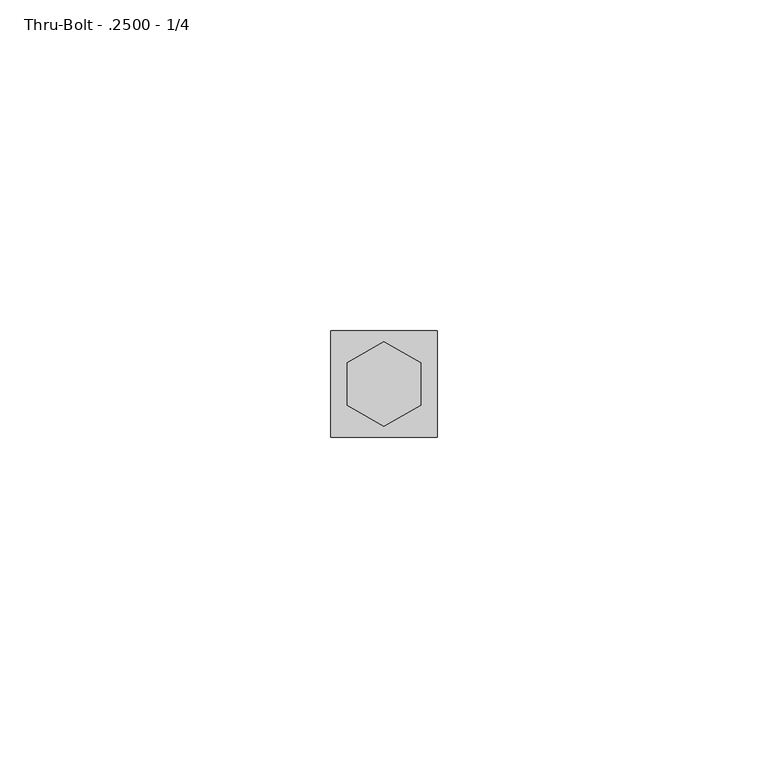
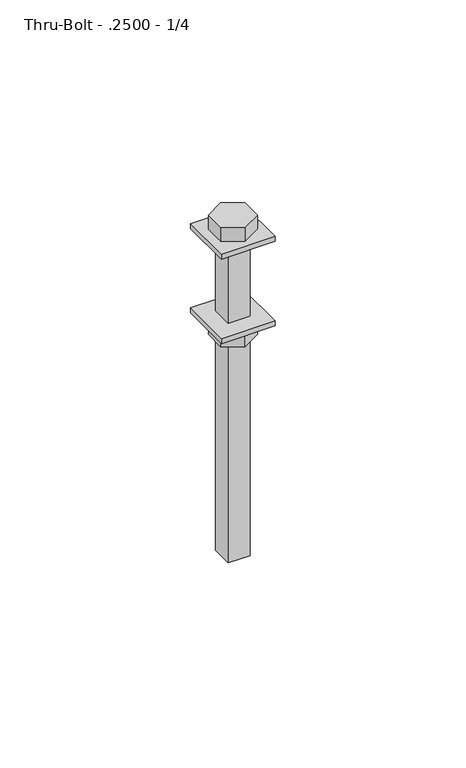
"""IFC4 building model written with IfcOpenShell, lengths in millimetres: fastener geometry, 060523 - W_P_C - Fastenings - Generic - SQUARE : Thru-Bolt - .2500 - 1/4."""

from ifc_helpers import new_model, si_unit, frame, origin, origin_with_axes, place, context, project, spatial, polyline, outline, extrude, source, transform, mapped, element, save


def thru_bolt_2500_1_4_f6ebfea6(model_context):
    return source(origin(), model_context, "Body", "SweptSolid", [
        extrude(outline(polyline([(-8.0645, -8.0645), (-8.0645, 8.0645), (8.0645, 8.0645), (8.0645, -8.0645), (-8.0645, -8.0645)])), origin_with_axes(), (0.0, 0.0, 1.0), 1.5875),
        extrude(outline(polyline([(-8.0645, -8.0645), (-8.0645, 8.0645), (8.0645, 8.0645), (8.0645, -8.0645), (-8.0645, -8.0645)])), frame((0.0, 0.0, -26.9875), z_axis=(0.0, 0.0, 1.0), x_axis=(1.0, 0.0, 0.0)), (0.0, 0.0, 1.0), 1.5875),
        extrude(outline(polyline([(-5.55625, -3.2079024), (-5.55625, 3.2079024), (0.0, 6.4158049), (5.55625, 3.2079024), (5.55625, -3.2079024), (0.0, -6.4158049), (-5.55625, -3.2079024)])), frame((0.0, 0.0, -31.75), z_axis=(0.0, 0.0, 1.0), x_axis=(1.0, 0.0, 0.0)), (0.0, 0.0, 1.0), 4.7625),
        extrude(outline(polyline([(-5.55625, 3.2079024), (0.0, 6.4158049), (5.55625, 3.2079024), (5.55625, -3.2079024), (0.0, -6.4158049), (-5.55625, -3.2079024), (-5.55625, 3.2079024)])), frame((0.0, 0.0, 1.5875), z_axis=(0.0, 0.0, 1.0), x_axis=(1.0, 0.0, 0.0)), (0.0, 0.0, 1.0), 4.7625),
        extrude(outline(polyline([(-3.302, 3.302), (3.302, 3.302), (3.302, -3.302), (-3.302, -3.302), (-3.302, 3.302)])), frame((0.0, 0.0, -101.6), z_axis=(0.0, 0.0, 1.0), x_axis=(1.0, 0.0, 0.0)), (0.0, 0.0, 1.0), 103.1875),
    ])


if __name__ == "__main__":
    model = new_model("IFC4")
    model_context = context("Model", 3, world=origin())
    ifc_project = project(units=[si_unit("LENGTHUNIT", "METRE", prefix="MILLI")], contexts=[model_context])
    site = spatial("IfcSite", under=ifc_project)
    building = spatial("IfcBuilding", under=site)
    placement = place(None, origin())
    thru_bolt_2500_1_4_shape = thru_bolt_2500_1_4_f6ebfea6(model_context)
    element("IfcFastener", 1, ObjectType="060523 - W_P_C - Fastenings - Generic - SQUARE : Thru-Bolt - .2500 - 1/4", at=placement, inside=building, context=model_context, shape_type="MappedRepresentation", body=[
        mapped(thru_bolt_2500_1_4_shape, transform((0.0, 0.0, 0.0), x_axis=(1.0, 0.0, 0.0), y_axis=(0.0, 1.0, 0.0), z_axis=(0.0, 0.0, 1.0))),
    ])
    save(model, "model.ifc")

# Revit data of these elements
# Type "060523 - W_P_C - Fastenings - Generic - SQUARE : Thru-Bolt - .2500 - 1/4"
#   Washer_Thickness = 0' - 0 1/16"
#   Washer Radius = 0' - 0.3175"
#   Washer Offset - Head = 0' - 0 1/16"
#   Washer Offset = 0' - 0 1/16"
#   Thickness_of_Substrate [instance default] = 0' - 1"
#   Side = 0' - 0.25293"
#   Radius = 0' - 0.13"
#   Length [instance default] = 0' - 4"
#   Head Size = 0' - 0 7/16"
#   Head Radius = 0' - 0 7/32"
#   Head Height = 0' - 0 3/16"
#   Double Diameter = 0' - 0.52"
#   Diameter = 0' - 0.26"
#   Default Elevation = 4' - 0"
#   Washer_Nut_Visibility = yes
#   Washer_Head_Visibility = yes
#   Round_Head_Visibility = no
#   Point Visibility = no
#   Nut_Visibility = yes
#   Hex_Head_Visiblilty = yes
#   Washer Material = none
#   Bolt Material (Size) = AT SILL - FASTENER AT 24" O.C.
# Element 1 (IfcFastener, "060523 - W_P_C - Fastenings - Generic - SQUARE : Thru-Bolt - .2500 - 1/4")
#   Materials on its faces: "AT SILL - FASTENER AT 24\" O.C."
# Materials
#   "AT SILL - FASTENER AT 24\" O.C.": class "Generic", colour RGB 120 120 120, transparency 0, Cost = 0
